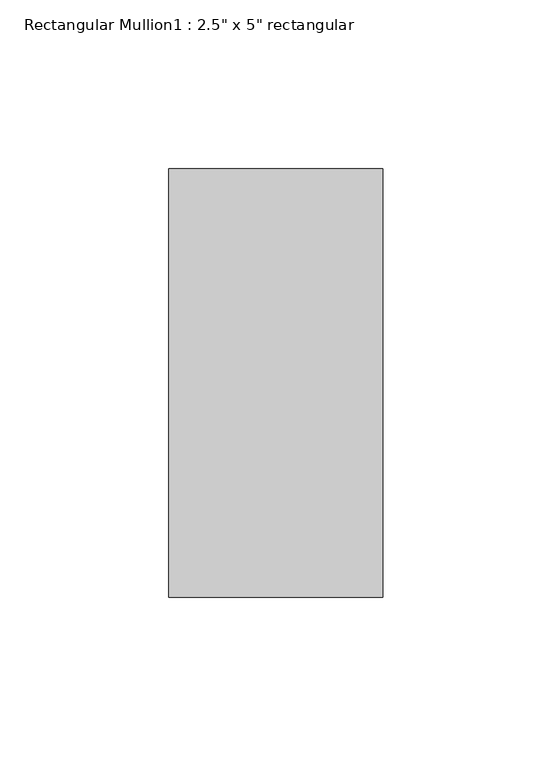
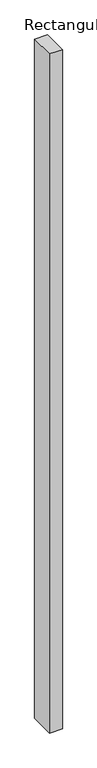
"""IFC4 building model written with IfcOpenShell, lengths in millimetres: member geometry."""

from ifc_helpers import new_model, si_unit, frame, origin, place, context, project, spatial, polyline, outline, extrude, source, transform, mapped, element, save


def member_5825c931(model_context):
    return source(origin(), model_context, "Body", "SweptSolid", [
        extrude(outline(polyline([(31.75, 63.5), (31.75, -63.5), (-31.75, -63.5), (-31.75, 63.5), (31.75, 63.5)])), frame((0.0, 0.0, -3556.0), z_axis=(0.0, 0.0, 1.0), x_axis=(1.0, 0.0, 0.0)), (0.0, 0.0, 1.0), 3556.0),
    ])


if __name__ == "__main__":
    model = new_model("IFC4")
    model_context = context("Model", 3, world=origin())
    ifc_project = project(units=[si_unit("LENGTHUNIT", "METRE", prefix="MILLI")], contexts=[model_context])
    site = spatial("IfcSite", under=ifc_project)
    building = spatial("IfcBuilding", under=site)
    placement = place(None, origin())
    member_shape = member_5825c931(model_context)
    element("IfcMember", 1, ObjectType="Rectangular Mullion1 : 2.5\" x 5\" rectangular", at=placement, inside=building, context=model_context, shape_type="MappedRepresentation", body=[
        mapped(member_shape, transform((0.0, 0.0, 0.0), x_axis=(1.0, 0.0, 0.0), y_axis=(0.0, 1.0, 0.0), z_axis=(0.0, 0.0, 1.0))),
    ])
    save(model, "model.ifc")

# Revit data of these elements
# Type "Rectangular Mullion1 : 2.5\" x 5\" rectangular"
#   built-in parameter 1007304 = 0.416667 (stored number, unit not read)
#   built-in parameter 1007301 = 0.104167 (stored number, unit not read)
#   built-in parameter 1007300 = 0.104167 (stored number, unit not read)
# Element 1 (IfcMember, "Rectangular Mullion1 : 2.5\" x 5\" rectangular")
#   Materials on its faces: "support-frame"
# Materials
#   "support-frame": class "Unassigned", colour RGB 233 233 233, transparency 0, Cost = 0
